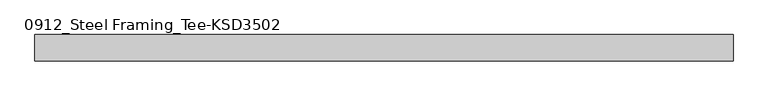
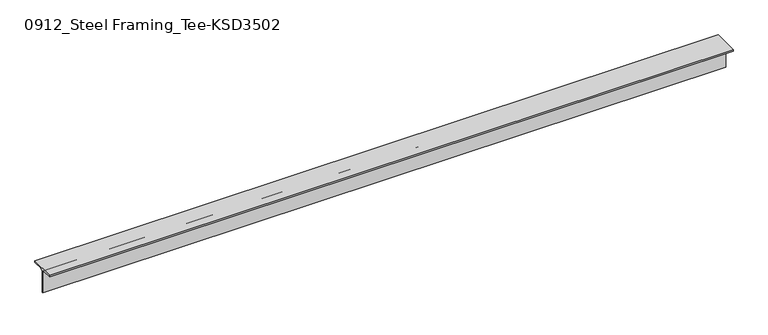
"""IFC4 building model written with IfcOpenShell, lengths in millimetres: member geometry, 0912_Steel Framing_Tee-KSD3502 : H_SB_ASB_CT-150x150x6.5x9."""

from ifc_helpers import new_model, si_unit, point, frame, frame_2d, origin, place, context, project, spatial, polyline, circle_curve, trimmed, segment, composite_curve, outline, extrude, source, transform, mapped, element, save


def member_0912_steel_framing_tee_ksd3502_ff4bf3cc(model_context):
    return source(origin(), model_context, "Body", "SweptSolid", [
        extrude(outline(composite_curve([segment(polyline([(-75.0, 75.0), (75.0, 75.0), (75.0, 66.0), (16.25, 66.0)]), True, "CONTINUOUS"), segment(trimmed(circle_curve(frame_2d((16.25, 53.0)), 13.0), [point((16.25, 66.0))], [point((3.25, 53.0))], True, "CARTESIAN"), True, "CONTINUOUS"), segment(polyline([(3.25, 53.0), (3.25, -75.0), (-3.25, -75.0), (-3.25, 53.0)]), True, "CONTINUOUS"), segment(trimmed(circle_curve(frame_2d((-16.25, 53.0)), 13.0), [point((-3.25, 53.0))], [point((-16.25, 66.0))], True, "CARTESIAN"), True, "CONTINUOUS"), segment(polyline([(-16.25, 66.0), (-75.0, 66.0), (-75.0, 75.0)]), True, "CONTINUOUS")], self_intersect=False)), frame((-1979.35, 0.0, 0.0), z_axis=(1.0, 0.0, 0.0), x_axis=(0.0, 1.0, 0.0)), (0.0, 0.0, 1.0), 3969.5),
    ])


if __name__ == "__main__":
    model = new_model("IFC4")
    model_context = context("Model", 3, world=origin())
    ifc_project = project(units=[si_unit("LENGTHUNIT", "METRE", prefix="MILLI")], contexts=[model_context])
    site = spatial("IfcSite", under=ifc_project)
    building = spatial("IfcBuilding", under=site)
    placement = place(None, origin())
    member_0912_steel_framing_tee_ksd3502_shape = member_0912_steel_framing_tee_ksd3502_ff4bf3cc(model_context)
    element("IfcMember", 1, ObjectType="0912_Steel Framing_Tee-KSD3502 : H_SB_ASB_CT-150x150x6.5x9", at=placement, inside=building, context=model_context, shape_type="MappedRepresentation", body=[
        mapped(member_0912_steel_framing_tee_ksd3502_shape, transform((0.0, 0.0, 0.0), x_axis=(1.0, 0.0, 0.0), y_axis=(0.0, 1.0, 0.0), z_axis=(0.0, 0.0, 1.0))),
    ])
    save(model, "model.ifc")

# Revit data of these elements
# Type "0912_Steel Framing_Tee-KSD3502 : H_SB_ASB_CT-150x150x6.5x9"
#   H_WM Code_1 = "S01AA003-00001 | Main Steel Structure Fabrication Work | Shelter/Building | Light Steel - Standard (30KG/M>Weight) | Material: (   )"
#   H_WM Code_2 = "S03AA029-00001 | Main Steel Structure Erection Work | Shelter/Building | Light Steel (30KG/M>Weight) | Material: (   )"
#   H_WM Code_3 = "S01AA010-00001 | Main Steel Structure Fabrication Work | Shelter/Building | Steel Painting/Coating | for Non-Fireproofed Steel Surface, Surface Preparation, Primer, Second & Final Coat | Material: (   )"
#   H_Q'ty Cal Type Tag = "SB-Q2"
#   Width = 15.0 cm
#   Web Thickness = 0.65 cm
#   Web Fillet = 1.3 cm
#   Section Area = 23.39 cm²
#   Perimeter = 0.60 m²/m
#   Nominal Weight = 18.40 kgf/m
#   Height = 15.0 cm
#   Flange Thickness = 0.9 cm
#   Centroid Vertical = 7.5 cm
#   Centroid Horizontal = 7.5 cm
#   Length [instance default] = 1.5000 m
#   Structural Material [instance default] = Steel, 45-345
#   Warping Constant = (empty or 0)
#   Torsional Moment of Inertia = 0
#   Section Name Key = ""
#   Plastic Modulus weak axis = 0
#   Plastic Modulus strong axis = 0
#   Moment of Inertia weak axis = 0
#   Moment of Inertia strong axis = 0
#   Elastic Modulus weak axis = 0
#   Elastic Modulus strong axis = 0
#   Bolt Spacing = 0
#   Assembly Code = ""
# Element 1 (IfcMember, "0912_Steel Framing_Tee-KSD3502 : H_SB_ASB_CT-150x150x6.5x9")
#   Structural Material = none
# Materials
#   "Steel, 45-345": class "Metal", colour RGB 189 187 185, transparency 0, Description = "Steel 345 MPa", Cost = 0
